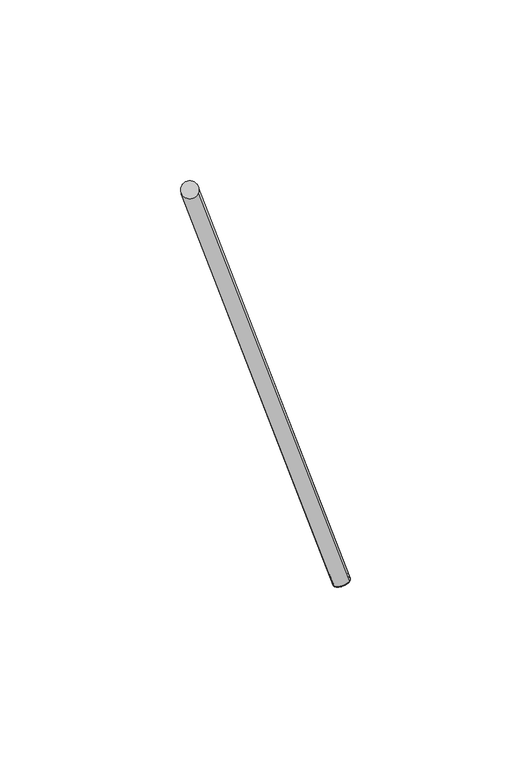
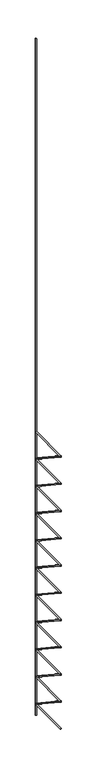
"""IFC4 building model written with IfcOpenShell, lengths in millimetres: proxy geometry, Vigota 1 (Pano 3) (Mf = 803)."""

from ifc_helpers import new_model, si_unit, point, frame, frame_2d, origin, origin_2d, place, context, project, spatial, circle_curve, trimmed, segment, composite_curve, outline, extrude, source, transform, mapped, element, save


def structural_framing_f0e1c358(model_context):
    return source(origin(), model_context, "Body", "SweptSolid", [
        extrude(outline(composite_curve([segment(trimmed(circle_curve(frame_2d((0.0, 108.0)), 2.5), [point((2.5, 108.0))], [point((-2.5, 108.0))], False, "CARTESIAN"), True, "CONTINUOUS"), segment(trimmed(circle_curve(frame_2d((0.0, 108.0)), 2.5), [point((-2.5, 108.0))], [point((2.5, 108.0))], False, "CARTESIAN"), True, "CONTINUOUS")], self_intersect=False)), frame((0.0, 0.0, 67.500535), z_axis=(0.0, 0.0, 1.0), x_axis=(1.0, 0.0, 0.0)), (0.0, 0.0, 1.0), 2980.0),
        extrude(outline(composite_curve([segment(trimmed(circle_curve(origin_2d(), 2.5), [point((2.5, 0.0))], [point((-2.5, 0.0))], False, "CARTESIAN"), True, "CONTINUOUS"), segment(trimmed(circle_curve(origin_2d(), 2.5), [point((-2.5, 0.0))], [point((2.5, 0.0))], False, "CARTESIAN"), True, "CONTINUOUS")], self_intersect=False)), frame((42.0, 0.0, 57.500535), z_axis=(-0.3218603428886276, 0.8276408817707567, 0.4598004898837537), x_axis=(0.8192319205108605, -3.936835275445103e-11, 0.5734623443750141)), (0.0, 0.0, 1.0), 130.491379),
        extrude(outline(composite_curve([segment(trimmed(circle_curve(origin_2d(), 2.5), [point((2.5, 0.0))], [point((-2.5, 0.0))], False, "CARTESIAN"), True, "CONTINUOUS"), segment(trimmed(circle_curve(origin_2d(), 2.5), [point((-2.5, 0.0))], [point((2.5, 0.0))], False, "CARTESIAN"), True, "CONTINUOUS")], self_intersect=False)), frame((0.0, 108.0, 117.500535), z_axis=(0.3218603428886276, -0.8276408817707567, 0.4598004898837537), x_axis=(0.8192319205108605, -3.936835275445103e-11, -0.5734623443750141)), (0.0, 0.0, 1.0), 130.491379),
        extrude(outline(composite_curve([segment(trimmed(circle_curve(origin_2d(), 2.5), [point((2.5, 0.0))], [point((-2.5, 0.0))], False, "CARTESIAN"), True, "CONTINUOUS"), segment(trimmed(circle_curve(origin_2d(), 2.5), [point((-2.5, 0.0))], [point((2.5, 0.0))], False, "CARTESIAN"), True, "CONTINUOUS")], self_intersect=False)), frame((42.0, 0.0, 177.500535), z_axis=(-0.3218603428886276, 0.8276408817707567, 0.4598004898837537), x_axis=(0.8192319205108605, -3.936835275445103e-11, 0.5734623443750141)), (0.0, 0.0, 1.0), 130.491379),
        extrude(outline(composite_curve([segment(trimmed(circle_curve(origin_2d(), 2.5), [point((2.5, 0.0))], [point((-2.5, 0.0))], False, "CARTESIAN"), True, "CONTINUOUS"), segment(trimmed(circle_curve(origin_2d(), 2.5), [point((-2.5, 0.0))], [point((2.5, 0.0))], False, "CARTESIAN"), True, "CONTINUOUS")], self_intersect=False)), frame((0.0, 108.0, 237.500535), z_axis=(0.3218603428886276, -0.8276408817707567, 0.4598004898837537), x_axis=(0.8192319205108605, -3.936835275445103e-11, -0.5734623443750141)), (0.0, 0.0, 1.0), 130.491379),
        extrude(outline(composite_curve([segment(trimmed(circle_curve(origin_2d(), 2.5), [point((2.5, 0.0))], [point((-2.5, 0.0))], False, "CARTESIAN"), True, "CONTINUOUS"), segment(trimmed(circle_curve(origin_2d(), 2.5), [point((-2.5, 0.0))], [point((2.5, 0.0))], False, "CARTESIAN"), True, "CONTINUOUS")], self_intersect=False)), frame((42.0, 0.0, 297.500535), z_axis=(-0.3218603428886276, 0.8276408817707567, 0.4598004898837537), x_axis=(0.8192319205108605, -3.936835275445103e-11, 0.5734623443750141)), (0.0, 0.0, 1.0), 130.491379),
        extrude(outline(composite_curve([segment(trimmed(circle_curve(origin_2d(), 2.5), [point((2.5, 0.0))], [point((-2.5, 0.0))], False, "CARTESIAN"), True, "CONTINUOUS"), segment(trimmed(circle_curve(origin_2d(), 2.5), [point((-2.5, 0.0))], [point((2.5, 0.0))], False, "CARTESIAN"), True, "CONTINUOUS")], self_intersect=False)), frame((0.0, 108.0, 357.500535), z_axis=(0.3218603428886276, -0.8276408817707567, 0.4598004898837537), x_axis=(0.8192319205108605, -3.936835275445103e-11, -0.5734623443750141)), (0.0, 0.0, 1.0), 130.491379),
        extrude(outline(composite_curve([segment(trimmed(circle_curve(origin_2d(), 2.5), [point((2.5, 0.0))], [point((-2.5, 0.0))], False, "CARTESIAN"), True, "CONTINUOUS"), segment(trimmed(circle_curve(origin_2d(), 2.5), [point((-2.5, 0.0))], [point((2.5, 0.0))], False, "CARTESIAN"), True, "CONTINUOUS")], self_intersect=False)), frame((42.0, 0.0, 417.500535), z_axis=(-0.3218603428886276, 0.8276408817707567, 0.4598004898837537), x_axis=(0.8192319205108605, -3.936835275445103e-11, 0.5734623443750141)), (0.0, 0.0, 1.0), 130.491379),
        extrude(outline(composite_curve([segment(trimmed(circle_curve(origin_2d(), 2.5), [point((2.5, 0.0))], [point((-2.5, 0.0))], False, "CARTESIAN"), True, "CONTINUOUS"), segment(trimmed(circle_curve(origin_2d(), 2.5), [point((-2.5, 0.0))], [point((2.5, 0.0))], False, "CARTESIAN"), True, "CONTINUOUS")], self_intersect=False)), frame((0.0, 108.0, 477.500535), z_axis=(0.3218603428886276, -0.8276408817707567, 0.4598004898837537), x_axis=(0.8192319205108605, -3.936835275445103e-11, -0.5734623443750141)), (0.0, 0.0, 1.0), 130.491379),
        extrude(outline(composite_curve([segment(trimmed(circle_curve(origin_2d(), 2.5), [point((2.5, 0.0))], [point((-2.5, 0.0))], False, "CARTESIAN"), True, "CONTINUOUS"), segment(trimmed(circle_curve(origin_2d(), 2.5), [point((-2.5, 0.0))], [point((2.5, 0.0))], False, "CARTESIAN"), True, "CONTINUOUS")], self_intersect=False)), frame((42.0, 0.0, 537.500535), z_axis=(-0.3218603428886276, 0.8276408817707567, 0.4598004898837537), x_axis=(0.8192319205108605, -3.936835275445103e-11, 0.5734623443750141)), (0.0, 0.0, 1.0), 130.491379),
        extrude(outline(composite_curve([segment(trimmed(circle_curve(origin_2d(), 2.5), [point((2.5, 0.0))], [point((-2.5, 0.0))], False, "CARTESIAN"), True, "CONTINUOUS"), segment(trimmed(circle_curve(origin_2d(), 2.5), [point((-2.5, 0.0))], [point((2.5, 0.0))], False, "CARTESIAN"), True, "CONTINUOUS")], self_intersect=False)), frame((0.0, 108.0, 597.500535), z_axis=(0.3218603428886276, -0.8276408817707567, 0.4598004898837537), x_axis=(0.8192319205108605, -3.936835275445103e-11, -0.5734623443750141)), (0.0, 0.0, 1.0), 130.491379),
        extrude(outline(composite_curve([segment(trimmed(circle_curve(origin_2d(), 2.5), [point((2.5, 0.0))], [point((-2.5, 0.0))], False, "CARTESIAN"), True, "CONTINUOUS"), segment(trimmed(circle_curve(origin_2d(), 2.5), [point((-2.5, 0.0))], [point((2.5, 0.0))], False, "CARTESIAN"), True, "CONTINUOUS")], self_intersect=False)), frame((42.0, 0.0, 657.500535), z_axis=(-0.3218603428886276, 0.8276408817707567, 0.4598004898837537), x_axis=(0.8192319205108605, -3.936835275445103e-11, 0.5734623443750141)), (0.0, 0.0, 1.0), 130.491379),
        extrude(outline(composite_curve([segment(trimmed(circle_curve(origin_2d(), 2.5), [point((2.5, 0.0))], [point((-2.5, 0.0))], False, "CARTESIAN"), True, "CONTINUOUS"), segment(trimmed(circle_curve(origin_2d(), 2.5), [point((-2.5, 0.0))], [point((2.5, 0.0))], False, "CARTESIAN"), True, "CONTINUOUS")], self_intersect=False)), frame((0.0, 108.0, 717.500535), z_axis=(0.3218603428886276, -0.8276408817707567, 0.4598004898837537), x_axis=(0.8192319205108605, -3.936835275445103e-11, -0.5734623443750141)), (0.0, 0.0, 1.0), 130.491379),
        extrude(outline(composite_curve([segment(trimmed(circle_curve(origin_2d(), 2.5), [point((2.5, 0.0))], [point((-2.5, 0.0))], False, "CARTESIAN"), True, "CONTINUOUS"), segment(trimmed(circle_curve(origin_2d(), 2.5), [point((-2.5, 0.0))], [point((2.5, 0.0))], False, "CARTESIAN"), True, "CONTINUOUS")], self_intersect=False)), frame((42.0, 0.0, 777.500535), z_axis=(-0.3218603428886276, 0.8276408817707567, 0.4598004898837537), x_axis=(0.8192319205108605, -3.936835275445103e-11, 0.5734623443750141)), (0.0, 0.0, 1.0), 130.491379),
        extrude(outline(composite_curve([segment(trimmed(circle_curve(origin_2d(), 2.5), [point((2.5, 0.0))], [point((-2.5, 0.0))], False, "CARTESIAN"), True, "CONTINUOUS"), segment(trimmed(circle_curve(origin_2d(), 2.5), [point((-2.5, 0.0))], [point((2.5, 0.0))], False, "CARTESIAN"), True, "CONTINUOUS")], self_intersect=False)), frame((0.0, 108.0, 837.500535), z_axis=(0.3218603428886276, -0.8276408817707567, 0.4598004898837537), x_axis=(0.8192319205108605, -3.936835275445103e-11, -0.5734623443750141)), (0.0, 0.0, 1.0), 130.491379),
        extrude(outline(composite_curve([segment(trimmed(circle_curve(origin_2d(), 2.5), [point((2.5, 0.0))], [point((-2.5, 0.0))], False, "CARTESIAN"), True, "CONTINUOUS"), segment(trimmed(circle_curve(origin_2d(), 2.5), [point((-2.5, 0.0))], [point((2.5, 0.0))], False, "CARTESIAN"), True, "CONTINUOUS")], self_intersect=False)), frame((42.0, 0.0, 897.500535), z_axis=(-0.3218603428886276, 0.8276408817707567, 0.4598004898837537), x_axis=(0.8192319205108605, -3.936835275445103e-11, 0.5734623443750141)), (0.0, 0.0, 1.0), 130.491379),
        extrude(outline(composite_curve([segment(trimmed(circle_curve(origin_2d(), 2.5), [point((2.5, 0.0))], [point((-2.5, 0.0))], False, "CARTESIAN"), True, "CONTINUOUS"), segment(trimmed(circle_curve(origin_2d(), 2.5), [point((-2.5, 0.0))], [point((2.5, 0.0))], False, "CARTESIAN"), True, "CONTINUOUS")], self_intersect=False)), frame((0.0, 108.0, 957.500535), z_axis=(0.3218603428886276, -0.8276408817707567, 0.4598004898837537), x_axis=(0.8192319205108605, -3.936835275445103e-11, -0.5734623443750141)), (0.0, 0.0, 1.0), 130.491379),
        extrude(outline(composite_curve([segment(trimmed(circle_curve(origin_2d(), 2.5), [point((2.5, 0.0))], [point((-2.5, 0.0))], False, "CARTESIAN"), True, "CONTINUOUS"), segment(trimmed(circle_curve(origin_2d(), 2.5), [point((-2.5, 0.0))], [point((2.5, 0.0))], False, "CARTESIAN"), True, "CONTINUOUS")], self_intersect=False)), frame((42.0, 0.0, 1017.500535), z_axis=(-0.3218603428886276, 0.8276408817707567, 0.4598004898837537), x_axis=(0.8192319205108605, -3.936835275445103e-11, 0.5734623443750141)), (0.0, 0.0, 1.0), 130.491379),
        extrude(outline(composite_curve([segment(trimmed(circle_curve(origin_2d(), 2.5), [point((2.5, 0.0))], [point((-2.5, 0.0))], False, "CARTESIAN"), True, "CONTINUOUS"), segment(trimmed(circle_curve(origin_2d(), 2.5), [point((-2.5, 0.0))], [point((2.5, 0.0))], False, "CARTESIAN"), True, "CONTINUOUS")], self_intersect=False)), frame((0.0, 108.0, 1077.500535), z_axis=(0.3218603428886276, -0.8276408817707567, 0.4598004898837537), x_axis=(0.8192319205108605, -3.936835275445103e-11, -0.5734623443750141)), (0.0, 0.0, 1.0), 130.491379),
        extrude(outline(composite_curve([segment(trimmed(circle_curve(origin_2d(), 2.5), [point((2.5, 0.0))], [point((-2.5, 0.0))], False, "CARTESIAN"), True, "CONTINUOUS"), segment(trimmed(circle_curve(origin_2d(), 2.5), [point((-2.5, 0.0))], [point((2.5, 0.0))], False, "CARTESIAN"), True, "CONTINUOUS")], self_intersect=False)), frame((42.0, 0.0, 1137.500535), z_axis=(-0.3218603428886276, 0.8276408817707567, 0.4598004898837537), x_axis=(0.8192319205108605, -3.936835275445103e-11, 0.5734623443750141)), (0.0, 0.0, 1.0), 130.491379),
        extrude(outline(composite_curve([segment(trimmed(circle_curve(origin_2d(), 2.5), [point((2.5, 0.0))], [point((-2.5, 0.0))], False, "CARTESIAN"), True, "CONTINUOUS"), segment(trimmed(circle_curve(origin_2d(), 2.5), [point((-2.5, 0.0))], [point((2.5, 0.0))], False, "CARTESIAN"), True, "CONTINUOUS")], self_intersect=False)), frame((0.0, 108.0, 1197.500535), z_axis=(0.3218603428886276, -0.8276408817707567, 0.4598004898837537), x_axis=(0.8192319205108605, -3.936835275445103e-11, -0.5734623443750141)), (0.0, 0.0, 1.0), 130.491379),
        extrude(outline(composite_curve([segment(trimmed(circle_curve(origin_2d(), 2.5), [point((2.5, 0.0))], [point((-2.5, 0.0))], False, "CARTESIAN"), True, "CONTINUOUS"), segment(trimmed(circle_curve(origin_2d(), 2.5), [point((-2.5, 0.0))], [point((2.5, 0.0))], False, "CARTESIAN"), True, "CONTINUOUS")], self_intersect=False)), frame((42.0, 0.0, 1257.500535), z_axis=(-0.3218603428886276, 0.8276408817707567, 0.4598004898837537), x_axis=(0.8192319205108605, -3.936835275445103e-11, 0.5734623443750141)), (0.0, 0.0, 1.0), 130.491379),
    ])


if __name__ == "__main__":
    model = new_model("IFC4")
    model_context = context("Model", 3, world=origin())
    ifc_project = project(units=[si_unit("LENGTHUNIT", "METRE", prefix="MILLI")], contexts=[model_context])
    site = spatial("IfcSite", under=ifc_project)
    building = spatial("IfcBuilding", under=site)
    placement = place(None, origin())
    structural_framing_shape = structural_framing_f0e1c358(model_context)
    element("IfcBuildingElementProxy", 1, Name="Vigota 1 (Pano 3) (Mf = 803)", ObjectType="Vigota 1 (Pano 3) (Mf = 803)", at=placement, inside=building, context=model_context, shape_type="MappedRepresentation", body=[
        mapped(structural_framing_shape, transform((0.0, 0.0, 0.0), x_axis=(1.0, 0.0, 0.0), y_axis=(0.0, 1.0, 0.0), z_axis=(0.0, 0.0, 1.0))),
    ])
    save(model, "model.ifc")

# Revit data of these elements
# Element 1 (IfcBuildingElementProxy, "Vigota 1 (Pano 3) (Mf = 803)")
#   Materials on its faces: "Aço", "Concreto armado"
# Materials
#   "Aço": class "Metal", colour RGB 120 120 120, transparency 0, Description = "Aço estrutural A36 grau, ASTM B, acabamento laminado", Cost = 0
#   "Concreto armado": class "Não atribuído", colour RGB 168 169 158, transparency 0
